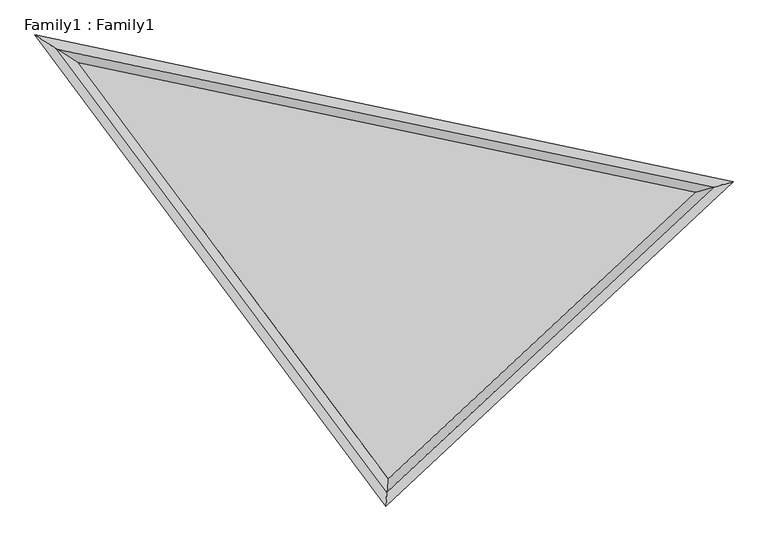
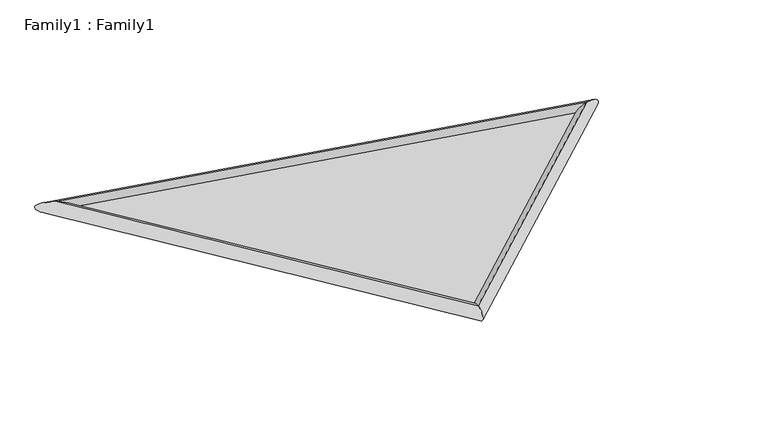
"""IFC4 building model written with IfcOpenShell, lengths in millimetres: proxy geometry, Family1 : Family1."""

from ifc_helpers import new_model, si_unit, frame, origin, origin_with_axes, place, context, project, spatial, polyline, ellipse_curve, outline, extrude, source, transform, mapped, element, save
from ifc_brep_helpers import cylinder_surface, advanced_brep


def family1_family1_343ef393(model_context):
    return source(origin(), model_context, "Body", "SolidModel", [
        extrude(outline(polyline([(933.8403475, -2221.7432357), (-2616.5762175, 2546.0379516), (4449.658321, 1059.646489), (933.8403475, -2221.7432357)])), origin_with_axes(), (0.0, 0.0, 1.0), 34.1328789),
        advanced_brep(
        [(933.8403475, -2221.7432357, 100.0), (933.8403475, -2221.7432357, -100.0), (-2616.5762175, 2546.0379516, -100.0), (-2616.5762175, 2546.0379516, 100.0), (4449.658321, 1059.646489, -100.0), (4449.658321, 1059.646489, 100.0)],
        [
            (0, 1, ellipse_curve(frame((933.8403475, -2221.7432357, 0.0), z_axis=(-0.9959620219312953, 0.08977555831364112, 0.0), x_axis=(-0.08977555831364105, -0.9959620219312952, 0.0)), 149.9582316, 100.0)),
            (1, 2),
            (2, 3, ellipse_curve(frame((-2616.5762175, 2546.0379516, 0.0), z_axis=(-0.5388087135139401, -0.8424281395118832, 0.0), x_axis=(0.8424281395118833, -0.5388087135139401, 0.0)), 282.598516, 100.0)),
            (3, 0),
            (1, 0, ellipse_curve(frame((933.8403475, -2221.7432357, 0.0), z_axis=(-0.9959620219312953, 0.08977555831364112, 0.0), x_axis=(-0.08977555831364105, -0.9959620219312952, 0.0)), 149.9582316, 100.0)),
            (3, 2, ellipse_curve(frame((-2616.5762175, 2546.0379516, 0.0), z_axis=(-0.5388087135139401, -0.8424281395118832, 0.0), x_axis=(0.8424281395118833, -0.5388087135139401, 0.0)), 282.598516, 100.0)),
            (2, 4),
            (4, 5, ellipse_curve(frame((4449.658321, 1059.646489, 0.0), z_axis=(-0.26846305195672526, 0.963289982162215, 0.0), x_axis=(-0.9632899821622151, -0.26846305195672515, 0.0)), 216.918065, 100.0)),
            (5, 3),
            (5, 4, ellipse_curve(frame((4449.658321, 1059.646489, 0.0), z_axis=(-0.26846305195672526, 0.963289982162215, 0.0), x_axis=(-0.9632899821622151, -0.26846305195672515, 0.0)), 216.918065, 100.0)),
            (4, 1),
            (0, 5),
        ],
        [
            cylinder_surface(frame((933.8403475, -2221.7432357, 0.0), z_axis=(0.597259784427102, -0.8020478476413311, 0.0), x_axis=(-0.8020478476413311, -0.597259784427102, 0.0)), 100.0),
            cylinder_surface(frame((-2616.5762175, 2546.0379516, 0.0), z_axis=(-0.9785843017837949, 0.2058464580757289, 0.0), x_axis=(0.2058464580757289, 0.9785843017837949, 0.0)), 100.0),
            cylinder_surface(frame((4449.658321, 1059.646489, 0.0), z_axis=(0.7310594568621078, 0.6823137625260681, 0.0), x_axis=(0.6823137625260681, -0.7310594568621078, 0.0)), 100.0),
        ],
        [
            (0, [[1, 2, 3, 4]]),
            (0, [[5, -4, 6, -2]]),
            (1, [[-3, 7, 8, 9]]),
            (1, [[-6, -9, 10, -7]]),
            (2, [[-8, 11, -1, 12]]),
            (2, [[-10, -12, -5, -11]]),
        ],
    ),
    ])


if __name__ == "__main__":
    model = new_model("IFC4")
    model_context = context("Model", 3, world=origin())
    ifc_project = project(units=[si_unit("LENGTHUNIT", "METRE", prefix="MILLI")], contexts=[model_context])
    site = spatial("IfcSite", under=ifc_project)
    building = spatial("IfcBuilding", under=site)
    placement = place(None, origin())
    family1_family1_shape = family1_family1_343ef393(model_context)
    element("IfcBuildingElementProxy", 1, Name="Family1 : Family1", ObjectType="Family1 : Family1", at=placement, inside=building, context=model_context, shape_type="MappedRepresentation", body=[
        mapped(family1_family1_shape, transform((0.0, 0.0, 0.0), x_axis=(1.0, 0.0, 0.0), y_axis=(0.0, 1.0, 0.0), z_axis=(0.0, 0.0, 1.0))),
    ])
    save(model, "model.ifc")

# Revit data of these elements
# Type "Family1 : Family1"
#   Default Elevation = 0
# Element 1 (IfcBuildingElementProxy, "Family1 : Family1")
#   Materials on its faces: "Glass"
# Materials
#   "Glass": class "Glass", colour RGB 0 128 192, transparency 0.9, Description = "Soda Lime Glass", Cost = 0
